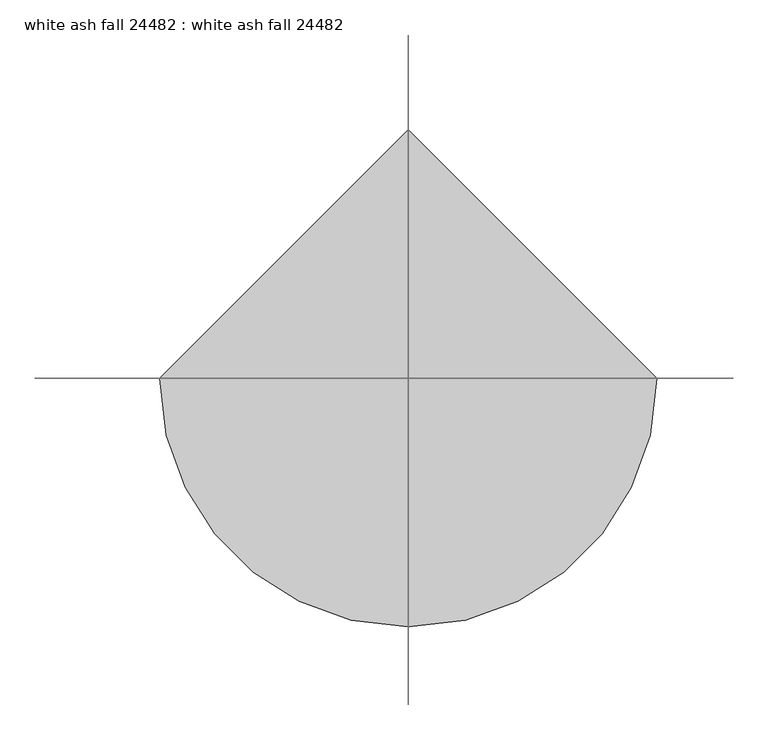
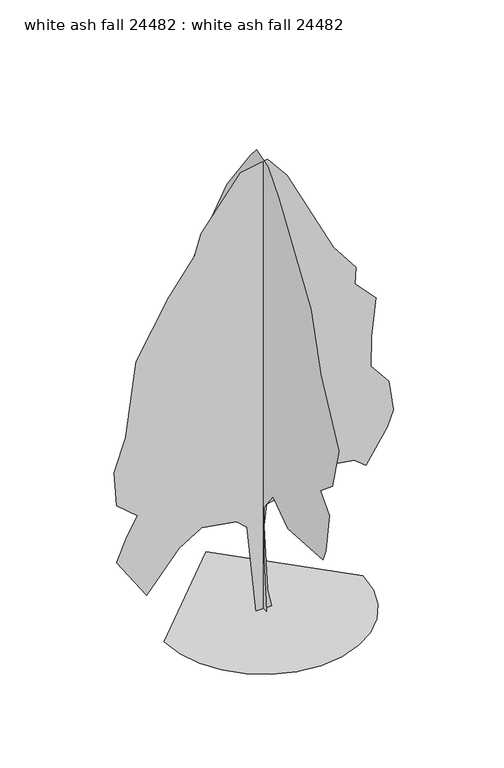
"""IFC4 building model written with IfcOpenShell, lengths in millimetres: proxy geometry, white ash fall 24482 : white ash fall 24482."""

import ifcopenshell
import ifcopenshell.guid

model = None  # the IFC model being written
_history = None  # IfcOwnerHistory: only IFC2X3 demands one
_inside = {}  # id of a spatial element -> (the spatial element, [elements in it])
_under = {}  # id of a project, library or spatial element -> (it, [spatial elements below it])
_declared = {}  # id of a project -> (the project, [libraries it declares])
_typed = {}  # id of a type object -> (the type object, [elements of that type])
_made_of = {}  # id of a material, layer set ... -> (it, [elements and type objects made of it])


def new_model(schema):
    """Start an empty IFC model of exactly this schema.

    Asked for "IFC4X3", IfcOpenShell would pick the latest addendum, in which some entities
    have other attributes; the version numbers below select the first issue.
    IFC2X3 requires an IfcOwnerHistory on every rooted entity: one is made here for all.
    """
    global model, _history
    if schema == "IFC4X3":
        model = ifcopenshell.file(schema_version=(4, 3, 0, 0))
    else:
        model = ifcopenshell.file(schema=schema)
    _inside.clear()
    _under.clear()
    _declared.clear()
    _typed.clear()
    _made_of.clear()
    _history = None
    if model.schema == "IFC2X3":
        org = make("IfcOrganization", Name="unknown")
        user = make(
            "IfcPersonAndOrganization",
            ThePerson=make("IfcPerson", FamilyName="unknown"),
            TheOrganization=org,
        )
        app = make(
            "IfcApplication",
            ApplicationDeveloper=org,
            Version="unknown",
            ApplicationFullName="unknown",
            ApplicationIdentifier="unknown",
        )
        _history = make(
            "IfcOwnerHistory",
            OwningUser=user,
            OwningApplication=app,
            ChangeAction="ADDED",
            CreationDate=0,
        )
    return model


def make(cls, **values):
    """One entity of the class cls with the attributes given. An attribute that is None is left unset."""
    return model.create_entity(
        cls, **{name: value for name, value in values.items() if value is not None}
    )


def rooted(cls, **values):
    """An entity with a GlobalId (a new one), such as an element, a storey or a relation."""
    return make(cls, GlobalId=ifcopenshell.guid.new(), OwnerHistory=_history, **values)


def si_unit(unit_type, name, prefix=None):
    """IfcSIUnit, for example si_unit("LENGTHUNIT", "METRE", prefix="MILLI")."""
    return make("IfcSIUnit", UnitType=unit_type, Prefix=prefix, Name=name)


def assignment(units):
    """IfcUnitAssignment: the units of a project."""
    return None if units is None else make("IfcUnitAssignment", Units=units)


def point(xyz):
    """IfcCartesianPoint."""
    return None if xyz is None else make("IfcCartesianPoint", Coordinates=xyz)


def direction(xyz):
    """IfcDirection."""
    return None if xyz is None else make("IfcDirection", DirectionRatios=xyz)


def frame(location, z_axis=None, x_axis=None):
    """IfcAxis2Placement3D, a coordinate frame: its origin and axes. An axis left out is left unset."""
    return make(
        "IfcAxis2Placement3D",
        Location=point(location),
        Axis=direction(z_axis),
        RefDirection=direction(x_axis),
    )


def origin():
    """The frame at (0, 0, 0) with its axes left unset."""
    return frame((0.0, 0.0, 0.0))


def place(relative_to, where):
    """IfcLocalPlacement: puts the frame where relative to a parent placement (None: the world)."""
    return make(
        "IfcLocalPlacement", PlacementRelTo=relative_to, RelativePlacement=where
    )


def context(
    kind, dimensions, precision=None, world=None, true_north=None, identifier=None
):
    """IfcGeometricRepresentationContext, for example the 3D "Model" context."""
    return make(
        "IfcGeometricRepresentationContext",
        ContextIdentifier=identifier,
        ContextType=kind,
        CoordinateSpaceDimension=dimensions,
        Precision=precision,
        WorldCoordinateSystem=world,
        TrueNorth=true_north,
    )


def project(units=None, contexts=None):
    """IfcProject with its units and contexts."""
    return rooted(
        "IfcProject",
        Name="project",
        RepresentationContexts=contexts,
        UnitsInContext=assignment(units),
    )


def spatial(cls, under=None, at=None, **own):
    """A site, building, storey or space (cls), placed at a placement, below another one or the project."""
    s = rooted(cls, ObjectPlacement=at, **own)
    if under is not None:
        _under.setdefault(under.id(), (under, []))[1].append(s)
    return s


def point_list(points):
    """IfcCartesianPointList2D or 3D."""
    cls = (
        "IfcCartesianPointList2D" if len(points[0]) == 2 else "IfcCartesianPointList3D"
    )
    return make(cls, CoordList=points)


def triangles(points, corners, closed=None, point_numbers=None):
    """IfcTriangulatedFaceSet: each triangle names its three corners, points numbered from 1."""
    return make(
        "IfcTriangulatedFaceSet",
        Coordinates=point_list(points),
        Closed=closed,
        CoordIndex=corners,
        PnIndex=point_numbers,
    )


def shape(context_of_items, identifier, shape_type, items):
    """IfcShapeRepresentation: the items that make up one representation, for example the "Body"."""
    return make(
        "IfcShapeRepresentation",
        ContextOfItems=context_of_items,
        RepresentationIdentifier=identifier,
        RepresentationType=shape_type,
        Items=items,
    )


def source(mapping_origin, context_of_items, identifier, shape_type, items):
    """IfcRepresentationMap: a shape defined once, which mapped items show again and again."""
    return make(
        "IfcRepresentationMap",
        MappingOrigin=mapping_origin,
        MappedRepresentation=shape(context_of_items, identifier, shape_type, items),
    )


def transform(
    local_origin,
    x_axis=None,
    y_axis=None,
    z_axis=None,
    scale=None,
    scale2=None,
    scale3=None,
    uniform=True,
):
    """IfcCartesianTransformationOperator3D, or its non-uniform kind. x_axis, y_axis, z_axis: its Axis1, 2, 3."""
    if uniform:
        return make(
            "IfcCartesianTransformationOperator3D",
            Axis1=direction(x_axis),
            Axis2=direction(y_axis),
            LocalOrigin=point(local_origin),
            Scale=scale,
            Axis3=direction(z_axis),
        )
    return make(
        "IfcCartesianTransformationOperator3DnonUniform",
        Axis1=direction(x_axis),
        Axis2=direction(y_axis),
        LocalOrigin=point(local_origin),
        Scale=scale,
        Axis3=direction(z_axis),
        Scale2=scale2,
        Scale3=scale3,
    )


def mapped(mapping_source, mapping_target):
    """IfcMappedItem: shows the shape of a source again, moved by a transform."""
    return make(
        "IfcMappedItem", MappingSource=mapping_source, MappingTarget=mapping_target
    )


def made_of(thing, what):
    """Note that an element or type object is made of a material, layer set ...; save() writes the relation."""
    if what is not None:
        _made_of.setdefault(what.id(), (what, []))[1].append(thing)
    return thing


def element(
    cls,
    number,
    at=None,
    inside=None,
    cuts=None,
    type_object=None,
    material=None,
    context=None,
    identifier="Body",
    shape_type=None,
    held_by="IfcProductDefinitionShape",
    body=None,
    shapes=None,
    **own,
):
    """One element of the class cls, such as IfcWall. Its Tag is "e" and its number.

    at: its placement. inside: the storey or other place that contains it. cuts: it is an
    opening in that element (IfcRelVoidsElement). A single representation is given by context,
    identifier, shape_type and body (its items); several are given by shapes. held_by: the class
    of the entity that holds the representations. save() writes the other relations.
    """
    e = rooted(cls, Tag="e%d" % number, ObjectPlacement=at, **own)
    if body is not None:
        shapes = [shape(context, identifier, shape_type, body)]
    if shapes is not None:
        e.Representation = make(held_by, Representations=shapes)
    if inside is not None:
        _inside.setdefault(inside.id(), (inside, []))[1].append(e)
    if cuts is not None:
        rooted(
            "IfcRelVoidsElement", RelatingBuildingElement=cuts, RelatedOpeningElement=e
        )
    if type_object is not None:
        _typed.setdefault(type_object.id(), (type_object, []))[1].append(e)
    return made_of(e, material)


def aggregate(whole, parts):
    """IfcRelAggregates: a whole, such as a stair, and the parts it consists of."""
    return rooted("IfcRelAggregates", RelatingObject=whole, RelatedObjects=parts)


def save(model, path):
    """Write the relations noted so far, then the file.

    IfcRelAggregates (storeys below a building ...), IfcRelContainedInSpatialStructure (elements
    in a storey), IfcRelDefinesByType, IfcRelAssociatesMaterial and IfcRelDeclares: one each for
    every whole, place, type object, material and project.
    """
    for whole, parts in _under.values():
        aggregate(whole, parts)
    for where, things in _inside.values():
        rooted(
            "IfcRelContainedInSpatialStructure",
            RelatedElements=things,
            RelatingStructure=where,
        )
    for kind, things in _typed.values():
        rooted("IfcRelDefinesByType", RelatedObjects=things, RelatingType=kind)
    for what, things in _made_of.values():
        rooted("IfcRelAssociatesMaterial", RelatedObjects=things, RelatingMaterial=what)
    for by, libraries in _declared.values():
        rooted("IfcRelDeclares", RelatingContext=by, RelatedDefinitions=libraries)
    model.write(path)


def white_ash_fall_24482_white_ash_fall_24482_ca342e74(model_context):
    return source(origin(), model_context, "Body", "Tessellation", [
        triangles([(-1903.1117432, 0.0, 0.0), (-1852.7994072, -436.0675326, 0.0), (-1709.5128044, -836.5267736, 0.0), (-1484.7201302, -1189.902079, 0.0), (-1189.902079, -1484.7201302, 0.0), (-836.5243029, -1709.5103336, 0.0), (-436.0675326, -1852.7994072, 0.0), (8.32e-05, -1903.1117432, 0.0), (436.0675326, -1852.7994072, 0.0), (836.5267736, -1709.5128044, 0.0), (1189.902079, -1484.7201302, 0.0), (1484.7201302, -1189.902079, 0.0), (1709.5103336, -836.5243029, 0.0), (1852.7994072, -436.0675326, 0.0), (1903.1117432, 0.0001664, 0.0), (-0.0002496, 1903.1117432, 0.0), (-6.4e-06, -107.924944, 0.0613456), (2.91e-05, -19.1547901, 1015.9932175), (6.03e-05, -22.4623803, 2068.4709812), (5.39e-05, -325.6028727, 2458.2394867), (1.45e-05, -807.5987429, 2100.6274487), (-5.27e-05, -1977.9757782, 2188.0796688), (-5.09e-05, -2067.0104599, 2427.1421116), (-3.51e-05, -2191.3969082, 3204.5680595), (-7.8e-06, -1895.979475, 3531.0600494), (-2.12e-05, -2284.6861267, 3857.5773285), (-9.2e-06, -2502.3617935, 4697.2004974), (6.13e-05, -1911.529398, 5878.860347), (0.0001153, -1572.9038464, 7015.6124725), (0.0002258, -512.181237, 8599.811705), (0.0002601, -154.5713246, 9035.1682709), (0.0002865, 234.1363626, 9144.0075577), (0.0002913, 433.9238045, 8906.4918228), (0.0003064, 1213.6790434, 7853.5084213), (0.0003087, 2239.8677868, 5877.6918137), (0.0003058, 2576.679641, 5106.6993393), (0.0002851, 2628.5718224, 4308.4785851), (0.0002675, 2473.0932312, 4028.6209579), (0.000235, 2395.3514648, 3095.7290634), (0.0002321, 2555.4707611, 2675.9174789), (0.0001966, 2115.4813385, 2364.9501228), (0.0001827, 2177.675798, 1774.1152565), (0.0001544, 1919.8426987, 1341.3319347), (0.0001354, 1726.7746868, 1089.9885555), (9.37e-05, 700.5858707, 1743.0180267), (9e-05, 514.0075064, 1991.7909233), (7.64e-05, 345.4377448, 1871.6004398), (4.67e-05, 163.0671178, 1239.2314808), (5.8e-06, 97.9767685, 0.0613703), (-139.7232302, 6.1e-06, 0.0682885), (-310.5051023, -0.0001955, 1753.6784225), (-510.5150233, -0.0002089, 1939.8629883), (-1184.5807468, -0.0001927, 2050.8713287), (-1618.5299858, -0.0001419, 1783.914513), (-2238.7425648, -2.84e-05, 1058.8988834), (-2814.0427689, -0.0001052, 1914.0565693), (-2611.9094673, -0.0001696, 2380.5051327), (-2409.7761658, -0.0002192, 2722.5774216), (-2814.0427689, -0.0002423, 3064.6393913), (-2860.6774223, -0.0003218, 3748.7636215), (-2642.9991394, -0.0004074, 4386.2279091), (-2440.8707794, -0.0005904, 5847.7703842), (-1817.4934227, -0.0007464, 6927.6777237), (-1321.3953609, -0.0008469, 7589.1960663), (-1197.0064419, -0.0009024, 8008.9820709), (-435.1404453, -0.0010506, 8972.9889267), (77.9529181, -0.0010842, 9066.2832321), (451.1119632, -0.0010468, 8615.3822662), (1343.785564, -0.0008745, 6842.8672028), (1771.7911251, -0.0008273, 6290.4422012), (1757.1683258, -0.0007869, 5956.609671), (2157.6860298, -0.0007547, 5539.8967346), (2072.4358555, -0.0006605, 4780.5631416), (2056.3779694, -0.0005886, 4183.7135262), (2399.5679226, -0.0005536, 3764.3083122), (2487.9397087, -0.0004852, 3157.9084076), (2379.1005672, -0.0004434, 2846.9613991), (1961.5166084, -0.0003491, 2209.4741478), (1741.621019, -0.0003618, 2396.0524395), (1104.141398, -0.0003453, 2491.7598244), (637.6903639, -0.0003117, 2380.5051327), (353.060281, -0.0002734, 2163.9953831), (54.4347815, -0.000252, 2094.0056145), (14.3638898, -0.0002002, 1674.2703335), (82.551847, -4.67e-05, 361.775047), (152.5283897, -6.7e-06, 0.0682758)], [[15, 16, 1], [14, 15, 1], [14, 1, 2], [13, 14, 2], [13, 2, 3], [13, 3, 4], [12, 13, 4], [11, 12, 4], [11, 4, 5], [11, 5, 6], [11, 6, 7], [11, 7, 8], [11, 8, 9], [11, 9, 10], [48, 49, 17], [48, 17, 18], [48, 18, 19], [47, 48, 19], [43, 44, 45], [42, 43, 45], [41, 42, 45], [41, 45, 46], [39, 40, 41], [31, 32, 33], [21, 22, 23], [21, 23, 24], [21, 24, 25], [20, 21, 25], [46, 47, 19], [30, 31, 33], [30, 33, 34], [29, 30, 34], [29, 34, 35], [28, 29, 35], [28, 35, 36], [28, 36, 37], [28, 37, 38], [27, 28, 38], [26, 27, 38], [25, 26, 38], [20, 25, 38], [20, 38, 39], [20, 39, 41], [20, 41, 46], [20, 46, 19], [85, 86, 50], [85, 50, 51], [84, 85, 51], [54, 55, 56], [54, 56, 57], [77, 78, 79], [83, 84, 51], [83, 51, 52], [54, 57, 58], [53, 54, 58], [66, 67, 68], [65, 66, 68], [65, 68, 69], [64, 65, 69], [63, 64, 69], [62, 63, 69], [61, 62, 69], [61, 69, 70], [61, 70, 71], [61, 71, 72], [61, 72, 73], [61, 73, 74], [60, 61, 74], [59, 60, 74], [58, 59, 74], [53, 58, 74], [52, 53, 74], [83, 52, 74], [82, 83, 74], [81, 82, 74], [80, 81, 74], [80, 74, 75], [79, 80, 75], [77, 79, 75], [77, 75, 76]], closed=False),
    ])


if __name__ == "__main__":
    model = new_model("IFC4")
    model_context = context("Model", 3, world=origin())
    ifc_project = project(units=[si_unit("LENGTHUNIT", "METRE", prefix="MILLI")], contexts=[model_context])
    site = spatial("IfcSite", under=ifc_project)
    building = spatial("IfcBuilding", under=site)
    placement = place(None, origin())
    white_ash_fall_24482_white_ash_fall_24482_shape = white_ash_fall_24482_white_ash_fall_24482_ca342e74(model_context)
    element("IfcBuildingElementProxy", 1, Name="white ash fall 24482 : white ash fall 24482", ObjectType="white ash fall 24482 : white ash fall 24482", at=placement, inside=building, context=model_context, shape_type="MappedRepresentation", body=[
        mapped(white_ash_fall_24482_white_ash_fall_24482_shape, transform((0.0, 0.0, 0.0), x_axis=(1.0, 0.0, 0.0), y_axis=(0.0, 1.0, 0.0), z_axis=(0.0, 0.0, 1.0))),
    ])
    save(model, "model.ifc")

# Revit data of these elements
# Type "white ash fall 24482 : white ash fall 24482"
#   built-in parameter 1005195 = "RPC-16-G1AF-G8PX-CFC7-2000-ST1L-LVER-AU"
#   Height = 0
